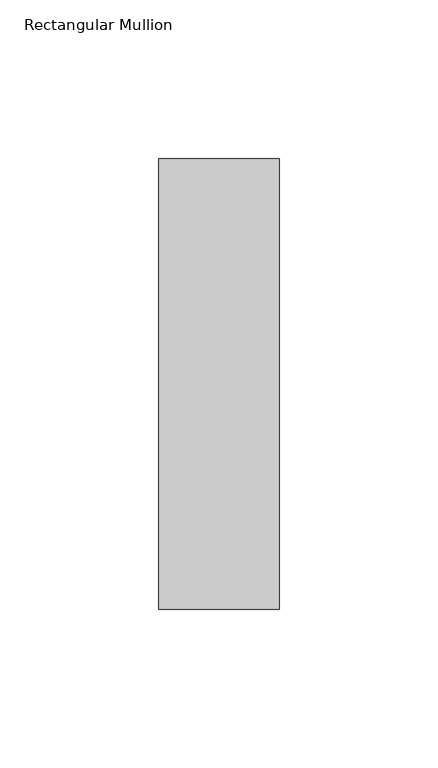
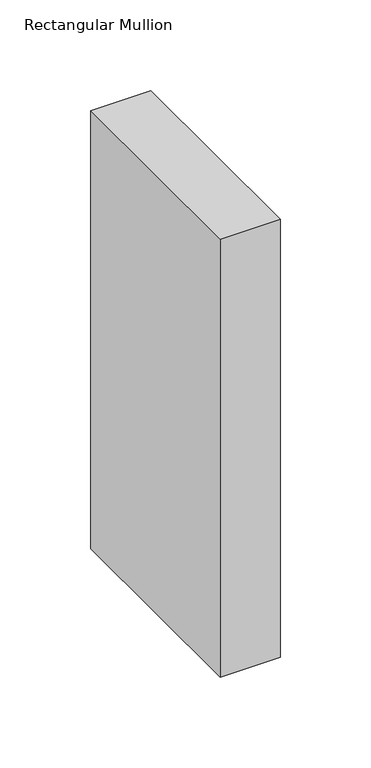
"""IFC4 building model written with IfcOpenShell, lengths in millimetres: member geometry, Rectangular Mullion : NLRS_21_CWM_hsb-regel 38x142_gen_rsf."""

from ifc_helpers import new_model, si_unit, frame, origin, place, context, project, spatial, polyline, outline, extrude, source, transform, mapped, element, save


def rectangular_mullion_45838a12(model_context):
    return source(origin(), model_context, "Body", "SweptSolid", [
        extrude(outline(polyline([(19.0, -71.0), (-19.0, -71.0), (-19.0, 71.0), (19.0, 71.0), (19.0, -71.0)])), frame((0.0, 0.0, -293.8441061), z_axis=(0.0, 0.0, 1.0), x_axis=(1.0, 0.0, 0.0)), (0.0, 0.0, 1.0), 293.8441061),
    ])


if __name__ == "__main__":
    model = new_model("IFC4")
    model_context = context("Model", 3, world=origin())
    ifc_project = project(units=[si_unit("LENGTHUNIT", "METRE", prefix="MILLI")], contexts=[model_context])
    site = spatial("IfcSite", under=ifc_project)
    building = spatial("IfcBuilding", under=site)
    placement = place(None, origin())
    rectangular_mullion_shape = rectangular_mullion_45838a12(model_context)
    element("IfcMember", 1, ObjectType="Rectangular Mullion : NLRS_21_CWM_hsb-regel 38x142_gen_rsf", at=placement, inside=building, context=model_context, shape_type="MappedRepresentation", body=[
        mapped(rectangular_mullion_shape, transform((0.0, 0.0, 0.0), x_axis=(1.0, 0.0, 0.0), y_axis=(0.0, 1.0, 0.0), z_axis=(0.0, 0.0, 1.0))),
    ])
    save(model, "model.ifc")

# Revit data of these elements
# Type "Rectangular Mullion : NLRS_21_CWM_hsb-regel 38x142_gen_rsf"
#   Export Type to IFC As = "IfcWall"
#   Type IfcGUID = "07M7mRoiH1CR8m_RSKIwpF"
#   Assembly Code = "21.10"
#   built-in parameter 1007322 = 0.465879 (stored number, unit not read)
#   built-in parameter 1007321 = 0.062336 (stored number, unit not read)
#   built-in parameter 1007320 = 0.062336 (stored number, unit not read)
# Element 1 (IfcMember, "Rectangular Mullion : NLRS_21_CWM_hsb-regel 38x142_gen_rsf")
#   Materials on its faces: "NLRS_i2_hout naaldhout vuren_gen_rsf"
# Materials
#   "NLRS_i2_hout naaldhout vuren_gen_rsf": class "I - Hout", colour RGB 234 199 147, transparency 0, Keynote = "i2", Manufacturer = "Revit Standards Foundation", URL = "www.revitstandards.org", Description = "hout vuren", Cost = 0
